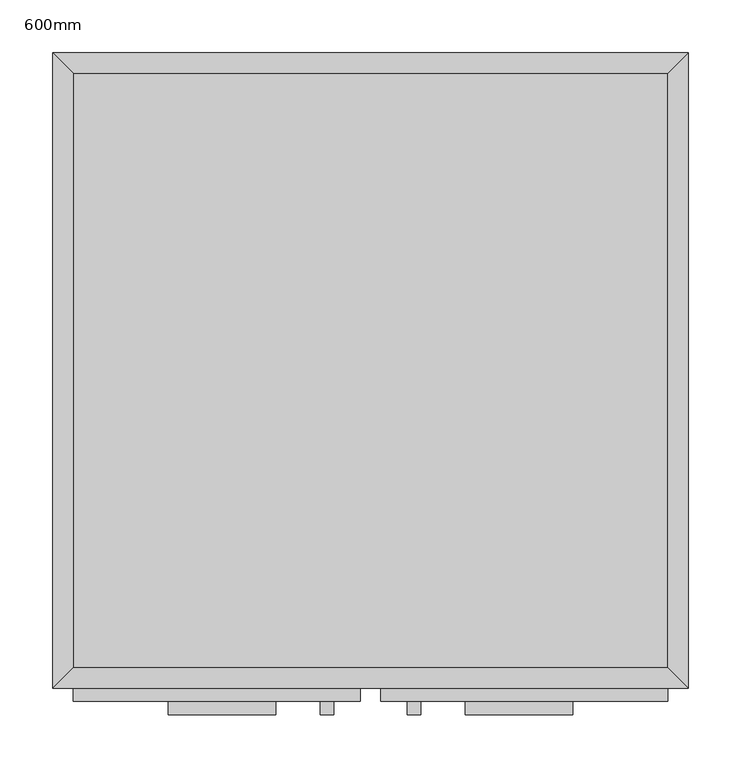
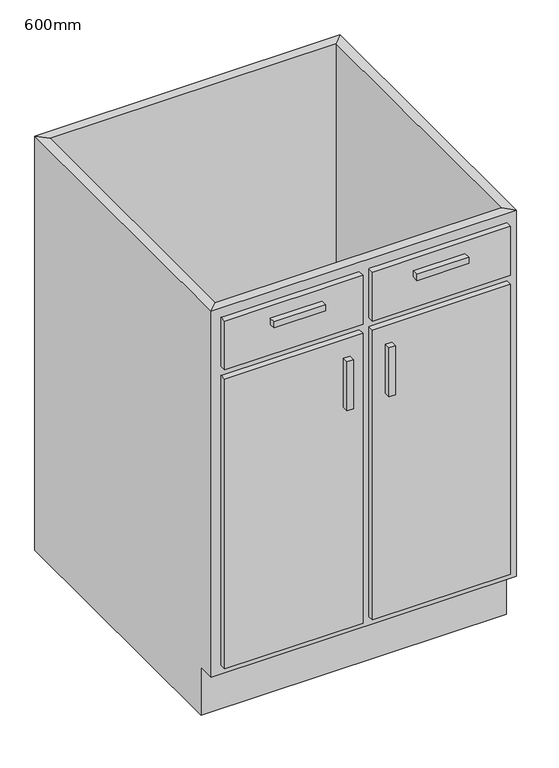
"""IFC4 building model written with IfcOpenShell, lengths in millimetres: furniture geometry, M_Base Cabinet-Double Door & 2 Drawer : 600mm."""

from ifc_helpers import new_model, si_unit, frame, origin, place, context, project, spatial, polyline, outline, extrude, faceted_brep, source, transform, mapped, element, save


def furniture_600mm_74c6c1e3(model_context):
    return source(origin(), model_context, "Body", "SolidModel", [
        faceted_brep([(299.6877049, -580.95, 860.0), (299.6877049, -580.95, 100.0), (-262.2122951, -580.95, 100.0), (-262.2122951, -580.95, 860.0), (-281.2622951, -600.0, 860.0), (318.7377049, -600.0, 860.0), (-281.2622951, -600.0, 100.0), (318.7377049, -600.0, 100.0), (-262.2122951, -565.0, 100.0), (-262.2122951, -19.05, 100.0), (-262.2122951, -19.05, 860.0), (-281.2622951, 0.0, 860.0), (-281.2622951, 0.0, 0.0), (-281.2622951, -565.0, 0.0), (-281.2622951, -565.0, 100.0), (299.6877049, -19.05, 100.0), (299.6877049, -19.05, 860.0), (318.7377049, 0.0, 860.0), (318.7377049, 0.0, 0.0), (299.6877049, -565.0, 100.0), (318.7377049, -565.0, 100.0), (318.7377049, -565.0, 0.0)], [[[0, 1, 2, 3]], [[0, 3, 4, 5]], [[5, 4, 6, 7]], [[2, 1, 7, 6]], [[3, 2, 8, 9, 10]], [[4, 3, 10, 11]], [[6, 4, 11, 12, 13, 14]], [[2, 6, 14, 8]], [[10, 9, 15, 16]], [[11, 10, 16, 17]], [[12, 11, 17, 18]], [[1, 0, 16, 15, 19]], [[0, 5, 17, 16]], [[5, 7, 20, 21, 18, 17]], [[7, 1, 19, 20]], [[8, 19, 15, 9]], [[18, 21, 13, 12]], [[13, 21, 20, 19, 8, 14]]]),
        extrude(outline(polyline([(-70.9372951, -625.4), (-172.5372951, -625.4), (-172.5372951, -612.7), (-70.9372951, -612.7), (-70.9372951, -625.4)])), frame((0.0, 0.0, 802.85), z_axis=(0.0, 0.0, 1.0), x_axis=(1.0, 0.0, 0.0)), (0.0, 0.0, 1.0), 12.7),
        extrude(outline(polyline([(210.0127049, -625.4), (108.4127049, -625.4), (108.4127049, -612.7), (210.0127049, -612.7), (210.0127049, -625.4)])), frame((0.0, 0.0, 802.85), z_axis=(0.0, 0.0, 1.0), x_axis=(1.0, 0.0, 0.0)), (0.0, 0.0, 1.0), 12.7),
        extrude(outline(polyline([(-16.1872951, -625.4), (-28.8872951, -625.4), (-28.8872951, -612.7), (-16.1872951, -612.7), (-16.1872951, -625.4)])), frame((0.0, 0.0, 580.6), z_axis=(0.0, 0.0, 1.0), x_axis=(1.0, 0.0, 0.0)), (0.0, 0.0, 1.0), 101.6),
        extrude(outline(polyline([(66.3627049, -625.4), (53.6627049, -625.4), (53.6627049, -612.7), (66.3627049, -612.7), (66.3627049, -625.4)])), frame((0.0, 0.0, 580.6), z_axis=(0.0, 0.0, 1.0), x_axis=(1.0, 0.0, 0.0)), (0.0, 0.0, 1.0), 101.6),
        extrude(outline(polyline([(9.2127049, -612.7), (-262.2122951, -612.7), (-262.2122951, -600.0), (9.2127049, -600.0), (9.2127049, -612.7)])), frame((0.0, 0.0, 739.35), z_axis=(0.0, 0.0, 1.0), x_axis=(1.0, 0.0, 0.0)), (0.0, 0.0, 1.0), 101.6),
        extrude(outline(polyline([(299.6877049, -612.7), (28.2627049, -612.7), (28.2627049, -600.0), (299.6877049, -600.0), (299.6877049, -612.7)])), frame((0.0, 0.0, 739.35), z_axis=(0.0, 0.0, 1.0), x_axis=(1.0, 0.0, 0.0)), (0.0, 0.0, 1.0), 101.6),
        extrude(outline(polyline([(9.2127049, -612.7), (-262.2122951, -612.7), (-262.2122951, -600.0), (9.2127049, -600.0), (9.2127049, -612.7)])), frame((0.0, 0.0, 119.05), z_axis=(0.0, 0.0, 1.0), x_axis=(1.0, 0.0, 0.0)), (0.0, 0.0, 1.0), 601.25),
        extrude(outline(polyline([(299.6877049, -612.7), (28.2627049, -612.7), (28.2627049, -600.0), (299.6877049, -600.0), (299.6877049, -612.7)])), frame((0.0, 0.0, 119.05), z_axis=(0.0, 0.0, 1.0), x_axis=(1.0, 0.0, 0.0)), (0.0, 0.0, 1.0), 601.25),
        extrude(outline(polyline([(299.6877049, -19.05), (299.6877049, -580.95), (-262.2122951, -580.95), (-262.2122951, -19.05), (299.6877049, -19.05)])), frame((0.0, 0.0, 100.0), z_axis=(0.0, 0.0, 1.0), x_axis=(1.0, 0.0, 0.0)), (0.0, 0.0, 1.0), 19.05),
    ])


if __name__ == "__main__":
    model = new_model("IFC4")
    model_context = context("Model", 3, world=origin())
    ifc_project = project(units=[si_unit("LENGTHUNIT", "METRE", prefix="MILLI")], contexts=[model_context])
    site = spatial("IfcSite", under=ifc_project)
    building = spatial("IfcBuilding", under=site)
    placement = place(None, origin())
    furniture_600mm_shape = furniture_600mm_74c6c1e3(model_context)
    element("IfcFurniture", 1, ObjectType="M_Base Cabinet-Double Door & 2 Drawer : 600mm", at=placement, inside=building, context=model_context, shape_type="MappedRepresentation", body=[
        mapped(furniture_600mm_shape, transform((0.0, 0.0, 0.0), x_axis=(1.0, 0.0, 0.0), y_axis=(0.0, 1.0, 0.0), z_axis=(0.0, 0.0, 1.0))),
    ])
    save(model, "model.ifc")

# Revit data of these elements
# Type "M_Base Cabinet-Double Door & 2 Drawer : 600mm"
#   Depth = 0.60 m
#   Height = 0.86 m
#   Plinth Depth = 0.035 m
#   Plinth Height = 0.10 m
#   Width = 0.60 m
#   Cabinet Material = none
#   Door/Drawer Material = none
#   Handle Material = Cabinets - Handles
# Element 1 (IfcFurniture, "M_Base Cabinet-Double Door & 2 Drawer : 600mm")
#   Materials on its faces: "Cabinets", "Cabinets - Handles"
# Materials
#   "Cabinets - Handles": class "Metal", colour RGB 57 57 57, transparency 0
#   "Cabinets": class "Miscellaneous", colour RGB 249 249 249, transparency 0
